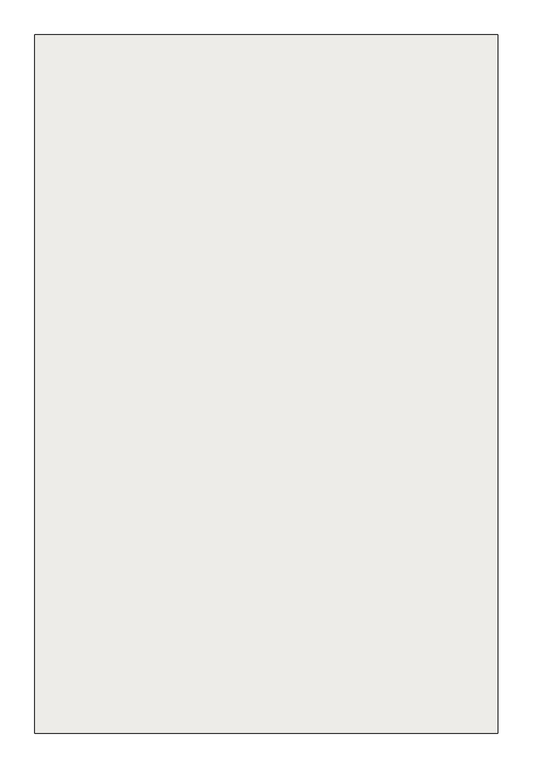
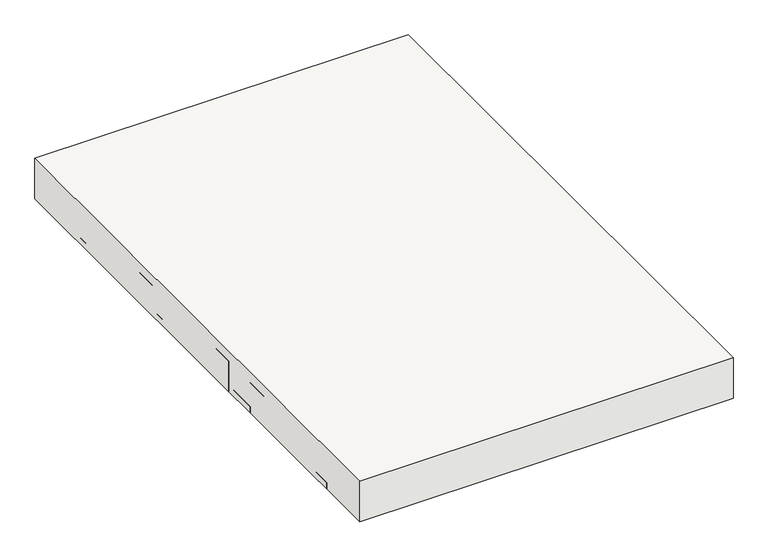
"""IFC4 building model written with IfcOpenShell, lengths in millimetres: slab geometry, Pano 12 (16 cm)."""

from ifc_helpers import new_model, si_unit, origin, origin_with_axes, place, context, project, spatial, polyline, outline, extrude, source, transform, mapped, element, save


def slab_42c2b4b9(model_context):
    return source(origin(), model_context, "Body", "SweptSolid", [
        extrude(outline(polyline([(2395.00107, 8235.0), (2395.00107, 10355.0), (3800.0, 10355.0), (3800.0, 8235.0), (2395.00107, 8235.0)])), origin_with_axes(), (0.0, 0.0, 1.0), 160.0),
        extrude(outline(polyline([(2395.00107, 9950.0), (2395.00107, 10090.0), (3800.0, 10090.0), (3800.0, 9950.0), (2395.00107, 9950.0)])), origin_with_axes(), (0.0, 0.0, 1.0), 24.0),
        extrude(outline(polyline([(3395.00107, 9090.0), (3395.00107, 9450.0), (3795.0, 9450.0), (3795.0, 9090.0), (3395.00107, 9090.0)])), origin_with_axes(), (0.0, 0.0, 1.0), 120.0),
        extrude(outline(polyline([(3395.00107, 8590.0), (3395.00107, 8950.0), (3795.0, 8950.0), (3795.0, 8590.0), (3395.00107, 8590.0)])), origin_with_axes(), (0.0, 0.0, 1.0), 120.0),
        extrude(outline(polyline([(2895.00107, 9090.0), (2895.00107, 9450.0), (3390.00107, 9450.0), (3390.00107, 9090.0), (2895.00107, 9090.0)])), origin_with_axes(), (0.0, 0.0, 1.0), 120.0),
        extrude(outline(polyline([(2395.00107, 8450.0), (2395.00107, 8590.0), (3800.0, 8590.0), (3800.0, 8450.0), (2395.00107, 8450.0)])), origin_with_axes(), (0.0, 0.0, 1.0), 24.0),
        extrude(outline(polyline([(2895.00107, 9590.0), (2895.00107, 9950.0), (3390.00107, 9950.0), (3390.00107, 9590.0), (2895.00107, 9590.0)])), origin_with_axes(), (0.0, 0.0, 1.0), 120.0),
        extrude(outline(polyline([(2395.00107, 9590.0), (2395.00107, 9950.0), (2890.00107, 9950.0), (2890.00107, 9590.0), (2395.00107, 9590.0)])), origin_with_axes(), (0.0, 0.0, 1.0), 120.0),
        extrude(outline(polyline([(2395.00107, 9090.0), (2395.00107, 9450.0), (2890.00107, 9450.0), (2890.00107, 9090.0), (2395.00107, 9090.0)])), origin_with_axes(), (0.0, 0.0, 1.0), 120.0),
        extrude(outline(polyline([(2395.00107, 9450.0), (2395.00107, 9590.0), (3800.0, 9590.0), (3800.0, 9450.0), (2395.00107, 9450.0)])), origin_with_axes(), (0.0, 0.0, 1.0), 24.0),
        extrude(outline(polyline([(3395.00107, 9590.0), (3395.00107, 9950.0), (3795.0, 9950.0), (3795.0, 9590.0), (3395.00107, 9590.0)])), origin_with_axes(), (0.0, 0.0, 1.0), 120.0),
        extrude(outline(polyline([(2895.00107, 8590.0), (2895.00107, 8950.0), (3390.00107, 8950.0), (3390.00107, 8590.0), (2895.00107, 8590.0)])), origin_with_axes(), (0.0, 0.0, 1.0), 120.0),
        extrude(outline(polyline([(2395.00107, 8950.0), (2395.00107, 9090.0), (3800.0, 9090.0), (3800.0, 8950.0), (2395.00107, 8950.0)])), origin_with_axes(), (0.0, 0.0, 1.0), 24.0),
        extrude(outline(polyline([(2395.00107, 8590.0), (2395.00107, 8950.0), (2890.00107, 8950.0), (2890.00107, 8590.0), (2395.00107, 8590.0)])), origin_with_axes(), (0.0, 0.0, 1.0), 120.0),
    ])


if __name__ == "__main__":
    model = new_model("IFC4")
    model_context = context("Model", 3, world=origin())
    ifc_project = project(units=[si_unit("LENGTHUNIT", "METRE", prefix="MILLI")], contexts=[model_context])
    site = spatial("IfcSite", under=ifc_project)
    building = spatial("IfcBuilding", under=site)
    placement = place(None, origin())
    slab_shape = slab_42c2b4b9(model_context)
    element("IfcSlab", 1, ObjectType="Pano 12 (16 cm)", at=placement, inside=building, context=model_context, shape_type="MappedRepresentation", body=[
        mapped(slab_shape, transform((0.0, 0.0, 0.0), x_axis=(1.0, 0.0, 0.0), y_axis=(0.0, 1.0, 0.0), z_axis=(0.0, 0.0, 1.0))),
    ])
    save(model, "model.ifc")

# Revit data of these elements
# Element 1 (IfcSlab, "Pano 12 (16 cm)")
#   Materials on its faces: "Molde de poliestireno", "Concreto armado", "RGB 168-169-158"
# Materials
#   "Molde de poliestireno": class "Não atribuído", colour RGB 255 255 255, transparency 0
#   "Concreto armado": class "Não atribuído", colour RGB 168 169 158, transparency 0
#   "RGB 168-169-158": class "Não atribuído", colour RGB 168 169 158, transparency 0
